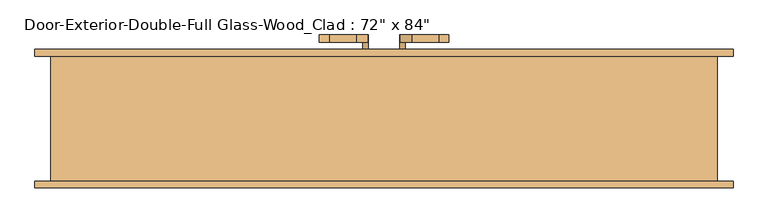
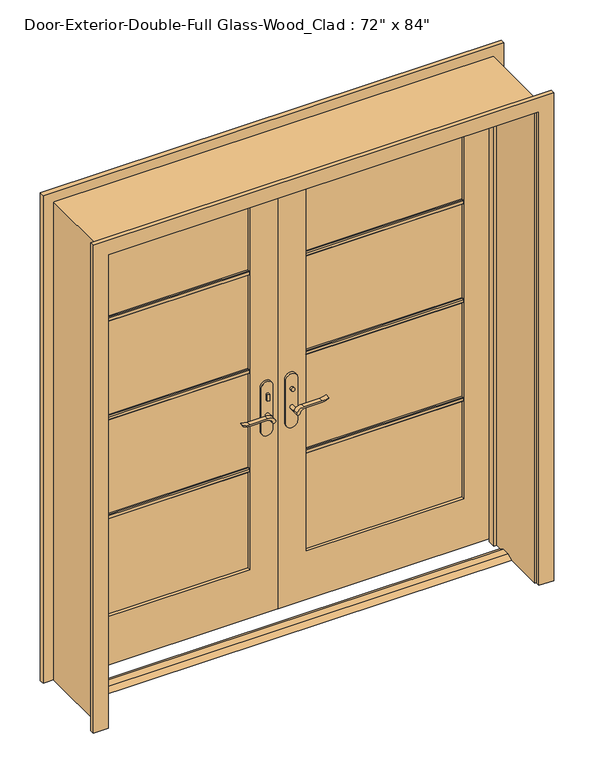
"""IFC4 building model written with IfcOpenShell, lengths in millimetres: door geometry."""

from ifc_helpers import new_model, si_unit, point, frame, frame_2d, origin, place, context, project, spatial, polyline, circle_curve, trimmed, segment, composite_curve, outline, extrude, faceted_brep, source, transform, mapped, element, save


def door_57570b86(model_context):
    return source(origin(), model_context, "Body", "SolidModel", [
        extrude(outline(polyline([(19.05, 12.7), (53.975, 12.7), (79.375, 0.0), (-6.35, 0.0), (19.05, 12.7)])), frame((-914.4, 0.0, 0.0), z_axis=(1.0, 0.0, 0.0), x_axis=(0.0, 1.0, 0.0)), (0.0, 0.0, 1.0), 1828.8),
        extrude(outline(polyline([(-47.4019111, 118.1125), (-57.4019111, 118.1125), (-57.4019111, 128.1125), (-47.4019111, 128.1125), (-47.4019111, 118.1125)])), frame((0.0, 0.0, 981.9), z_axis=(0.0, 0.0, 1.0), x_axis=(1.0, 0.0, 0.0)), (0.0, 0.0, 1.0), 30.0),
        extrude(outline(composite_curve([segment(trimmed(circle_curve(frame_2d((996.9, -52.4019111)), 8.0), [point((996.9, -60.4019111))], [point((996.9, -44.4019111))], False, "CARTESIAN"), True, "CONTINUOUS"), segment(trimmed(circle_curve(frame_2d((996.9, -52.4019111)), 8.0), [point((996.9, -44.4019111))], [point((996.9, -60.4019111))], False, "CARTESIAN"), True, "CONTINUOUS")], self_intersect=False)), frame((0.0, 183.0375, 0.0), z_axis=(0.0, 1.0, 0.0), x_axis=(0.0, 0.0, 1.0)), (0.0, 0.0, 1.0), 10.0),
        extrude(outline(composite_curve([segment(trimmed(circle_curve(frame_2d((897.1555521, -76.0694241)), 37.2832219), [point((919.0523287, -45.8937749))], [point((934.4, -77.7693445))], False, "CARTESIAN"), True, "CONTINUOUS"), segment(polyline([(934.4, -77.7693445), (934.4, -154.045502)]), True, "CONTINUOUS"), segment(trimmed(circle_curve(frame_2d((1017.6850638, -153.9791202)), 83.2850902), [point((934.4, -154.045502))], [point((939.4, -182.4019111))], True, "CARTESIAN"), True, "CONTINUOUS"), segment(polyline([(939.4, -182.4019111), (936.6135558, -182.4019111)]), True, "CONTINUOUS"), segment(trimmed(circle_curve(frame_2d((986.6709207, -150.4622499)), 59.3791355), [point((936.6135558, -182.4019111))], [point((927.4, -154.045502))], False, "CARTESIAN"), True, "CONTINUOUS"), segment(polyline([(927.4, -154.045502), (927.4, -77.7881013)]), True, "CONTINUOUS"), segment(trimmed(circle_curve(frame_2d((909.2738613, -77.7881013)), 18.1261387), [point((927.4, -77.7881013))], [point((914.4, -60.4019111))], True, "CARTESIAN"), True, "CONTINUOUS"), segment(trimmed(circle_curve(frame_2d((914.4, -52.4019111)), 8.0), [point((914.4, -60.4019111))], [point((919.0523287, -45.8937749))], False, "CARTESIAN"), True, "CONTINUOUS")], self_intersect=False)), frame((0.0, 78.1125, 0.0), z_axis=(0.0, 1.0, 0.0), x_axis=(0.0, 0.0, 1.0)), (0.0, 0.0, 1.0), 20.0),
        extrude(outline(composite_curve([segment(trimmed(circle_curve(frame_2d((914.4, -52.4019111)), 8.0), [point((914.3999903, -60.4019111))], [point((919.0523287, -45.8937749))], False, "CARTESIAN"), True, "CONTINUOUS"), segment(trimmed(circle_curve(frame_2d((897.1555521, -76.0694241)), 37.2832219), [point((919.0523287, -45.8937749))], [point((934.4, -77.7693445))], False, "CARTESIAN"), True, "CONTINUOUS"), segment(polyline([(934.4, -77.7693445), (934.4, -154.045502)]), True, "CONTINUOUS"), segment(trimmed(circle_curve(frame_2d((1017.6850638, -153.9791202)), 83.2850902), [point((934.4, -154.045502))], [point((939.4, -182.4019111))], True, "CARTESIAN"), True, "CONTINUOUS"), segment(polyline([(939.4, -182.4019111), (936.6135558, -182.4019111)]), True, "CONTINUOUS"), segment(trimmed(circle_curve(frame_2d((986.6709207, -150.4622499)), 59.3791355), [point((936.6135558, -182.4019111))], [point((927.4, -154.045502))], False, "CARTESIAN"), True, "CONTINUOUS"), segment(polyline([(927.4, -154.045502), (927.4, -77.788099)]), True, "CONTINUOUS"), segment(trimmed(circle_curve(frame_2d((909.2738682, -77.788099)), 18.1261318), [point((927.4, -77.788099))], [point((914.3999903, -60.4019111))], True, "CARTESIAN"), True, "CONTINUOUS")], self_intersect=False)), frame((0.0, 213.0375, 0.0), z_axis=(0.0, 1.0, 0.0), x_axis=(0.0, 0.0, 1.0)), (0.0, 0.0, 1.0), 20.0),
        extrude(outline(composite_curve([segment(trimmed(circle_curve(frame_2d((914.4, -52.4019111)), 8.0), [point((914.4, -60.4019111))], [point((914.4, -44.4019111))], False, "CARTESIAN"), True, "CONTINUOUS"), segment(trimmed(circle_curve(frame_2d((914.4, -52.4019111)), 8.0), [point((914.4, -44.4019111))], [point((914.4, -60.4019111))], False, "CARTESIAN"), True, "CONTINUOUS")], self_intersect=False)), frame((0.0, 98.1125, 0.0), z_axis=(0.0, 1.0, 0.0), x_axis=(0.0, 0.0, 1.0)), (0.0, 0.0, 1.0), 30.0),
        extrude(outline(composite_curve([segment(trimmed(circle_curve(frame_2d((914.4, -52.4019111)), 8.0), [point((914.4, -60.4019111))], [point((914.4, -44.4019111))], False, "CARTESIAN"), True, "CONTINUOUS"), segment(trimmed(circle_curve(frame_2d((914.4, -52.4019111)), 8.0), [point((914.4, -44.4019111))], [point((914.4, -60.4019111))], False, "CARTESIAN"), True, "CONTINUOUS")], self_intersect=False)), frame((0.0, 183.0375, 0.0), z_axis=(0.0, 1.0, 0.0), x_axis=(0.0, 0.0, 1.0)), (0.0, 0.0, 1.0), 30.0),
        extrude(outline(composite_curve([segment(polyline([(844.4, -27.4019111), (1039.4, -27.4019111)]), True, "CONTINUOUS"), segment(trimmed(circle_curve(frame_2d((1039.4, -52.4019111)), 25.0), [point((1039.4, -27.4019111))], [point((1039.4, -77.4019111))], False, "CARTESIAN"), True, "CONTINUOUS"), segment(polyline([(1039.4, -77.4019111), (844.4, -77.4019111)]), True, "CONTINUOUS"), segment(trimmed(circle_curve(frame_2d((844.4, -52.4019111)), 25.0), [point((844.4, -77.4019111))], [point((844.4, -27.4019111))], False, "CARTESIAN"), True, "CONTINUOUS")], self_intersect=False)), frame((0.0, 128.1125, 0.0), z_axis=(0.0, 1.0, 0.0), x_axis=(0.0, 0.0, 1.0)), (0.0, 0.0, 1.0), 10.0),
        extrude(outline(composite_curve([segment(polyline([(844.4, -27.4019111), (1039.4, -27.4019111)]), True, "CONTINUOUS"), segment(trimmed(circle_curve(frame_2d((1039.4, -52.4019111)), 25.0), [point((1039.4, -27.4019111))], [point((1039.4, -77.4019111))], False, "CARTESIAN"), True, "CONTINUOUS"), segment(polyline([(1039.4, -77.4019111), (844.4, -77.4019111)]), True, "CONTINUOUS"), segment(trimmed(circle_curve(frame_2d((844.4, -52.4019111)), 25.0), [point((844.4, -77.4019111))], [point((844.4, -27.4019111))], False, "CARTESIAN"), True, "CONTINUOUS")], self_intersect=False)), frame((0.0, 173.0375, 0.0), z_axis=(0.0, 1.0, 0.0), x_axis=(0.0, 0.0, 1.0)), (0.0, 0.0, 1.0), 10.0),
        extrude(outline(polyline([(47.3875, 193.0375), (57.3875, 193.0375), (57.3875, 183.0375), (47.3875, 183.0375), (47.3875, 193.0375)])), frame((0.0, 0.0, 981.9), z_axis=(0.0, 0.0, 1.0), x_axis=(1.0, 0.0, 0.0)), (0.0, 0.0, 1.0), 30.0),
        extrude(outline(composite_curve([segment(trimmed(circle_curve(frame_2d((996.9, 52.3875)), 8.0), [point((996.9, 60.3875))], [point((996.9, 44.3875))], False, "CARTESIAN"), True, "CONTINUOUS"), segment(trimmed(circle_curve(frame_2d((996.9, 52.3875)), 8.0), [point((996.9, 44.3875))], [point((996.9, 60.3875))], False, "CARTESIAN"), True, "CONTINUOUS")], self_intersect=False)), frame((0.0, 118.1125, 0.0), z_axis=(0.0, 1.0, 0.0), x_axis=(0.0, 0.0, 1.0)), (0.0, 0.0, 1.0), 10.0),
        extrude(outline(composite_curve([segment(trimmed(circle_curve(frame_2d((914.4, 52.3875)), 8.0), [point((919.0523287, 45.8793637))], [point((914.4, 60.3875))], False, "CARTESIAN"), True, "CONTINUOUS"), segment(trimmed(circle_curve(frame_2d((909.2738613, 77.7736901)), 18.1261387), [point((914.4, 60.3875))], [point((927.4, 77.7736901))], True, "CARTESIAN"), True, "CONTINUOUS"), segment(polyline([(927.4, 77.7736901), (927.4, 154.0310909)]), True, "CONTINUOUS"), segment(trimmed(circle_curve(frame_2d((986.6709207, 150.4478388)), 59.3791355), [point((927.4, 154.0310909))], [point((936.6135558, 182.3875))], False, "CARTESIAN"), True, "CONTINUOUS"), segment(polyline([(936.6135558, 182.3875), (939.4, 182.3875)]), True, "CONTINUOUS"), segment(trimmed(circle_curve(frame_2d((1017.6850638, 153.9647091)), 83.2850902), [point((939.4, 182.3875))], [point((934.4, 154.0310909))], True, "CARTESIAN"), True, "CONTINUOUS"), segment(polyline([(934.4, 154.0310909), (934.4, 77.7549333)]), True, "CONTINUOUS"), segment(trimmed(circle_curve(frame_2d((897.1555521, 76.0550129)), 37.2832219), [point((934.4, 77.7549333))], [point((919.0523287, 45.8793637))], False, "CARTESIAN"), True, "CONTINUOUS")], self_intersect=False)), frame((0.0, 213.0375, 0.0), z_axis=(0.0, 1.0, 0.0), x_axis=(0.0, 0.0, 1.0)), (0.0, 0.0, 1.0), 20.0),
        extrude(outline(composite_curve([segment(trimmed(circle_curve(frame_2d((909.2738682, 77.7736878)), 18.1261318), [point((914.3999903, 60.3875))], [point((927.4, 77.7736878))], True, "CARTESIAN"), True, "CONTINUOUS"), segment(polyline([(927.4, 77.7736878), (927.4, 154.0310909)]), True, "CONTINUOUS"), segment(trimmed(circle_curve(frame_2d((986.6709207, 150.4478388)), 59.3791355), [point((927.4, 154.0310909))], [point((936.6135558, 182.3875))], False, "CARTESIAN"), True, "CONTINUOUS"), segment(polyline([(936.6135558, 182.3875), (939.4, 182.3875)]), True, "CONTINUOUS"), segment(trimmed(circle_curve(frame_2d((1017.6850638, 153.9647091)), 83.2850902), [point((939.4, 182.3875))], [point((934.4, 154.0310909))], True, "CARTESIAN"), True, "CONTINUOUS"), segment(polyline([(934.4, 154.0310909), (934.4, 77.7549333)]), True, "CONTINUOUS"), segment(trimmed(circle_curve(frame_2d((897.1555521, 76.0550129)), 37.2832219), [point((934.4, 77.7549333))], [point((919.0523287, 45.8793637))], False, "CARTESIAN"), True, "CONTINUOUS"), segment(trimmed(circle_curve(frame_2d((914.4, 52.3875)), 8.0), [point((919.0523287, 45.8793637))], [point((914.3999903, 60.3875))], False, "CARTESIAN"), True, "CONTINUOUS")], self_intersect=False)), frame((0.0, 78.1125, 0.0), z_axis=(0.0, 1.0, 0.0), x_axis=(0.0, 0.0, 1.0)), (0.0, 0.0, 1.0), 20.0),
        extrude(outline(composite_curve([segment(trimmed(circle_curve(frame_2d((914.4, 52.3875)), 8.0), [point((914.4, 60.3875))], [point((914.4, 44.3875))], False, "CARTESIAN"), True, "CONTINUOUS"), segment(trimmed(circle_curve(frame_2d((914.4, 52.3875)), 8.0), [point((914.4, 44.3875))], [point((914.4, 60.3875))], False, "CARTESIAN"), True, "CONTINUOUS")], self_intersect=False)), frame((0.0, 183.0375, 0.0), z_axis=(0.0, 1.0, 0.0), x_axis=(0.0, 0.0, 1.0)), (0.0, 0.0, 1.0), 30.0),
        extrude(outline(composite_curve([segment(trimmed(circle_curve(frame_2d((914.4, 52.3875)), 8.0), [point((914.4, 60.3875))], [point((914.4, 44.3875))], False, "CARTESIAN"), True, "CONTINUOUS"), segment(trimmed(circle_curve(frame_2d((914.4, 52.3875)), 8.0), [point((914.4, 44.3875))], [point((914.4, 60.3875))], False, "CARTESIAN"), True, "CONTINUOUS")], self_intersect=False)), frame((0.0, 98.1125, 0.0), z_axis=(0.0, 1.0, 0.0), x_axis=(0.0, 0.0, 1.0)), (0.0, 0.0, 1.0), 30.0),
        extrude(outline(composite_curve([segment(trimmed(circle_curve(frame_2d((844.4, 52.3875)), 25.0), [point((844.4, 27.3875))], [point((844.4, 77.3875))], False, "CARTESIAN"), True, "CONTINUOUS"), segment(polyline([(844.4, 77.3875), (1039.4, 77.3875)]), True, "CONTINUOUS"), segment(trimmed(circle_curve(frame_2d((1039.4, 52.3875)), 25.0), [point((1039.4, 77.3875))], [point((1039.4, 27.3875))], False, "CARTESIAN"), True, "CONTINUOUS"), segment(polyline([(1039.4, 27.3875), (844.4, 27.3875)]), True, "CONTINUOUS")], self_intersect=False)), frame((0.0, 173.0375, 0.0), z_axis=(0.0, 1.0, 0.0), x_axis=(0.0, 0.0, 1.0)), (0.0, 0.0, 1.0), 10.0),
        extrude(outline(composite_curve([segment(trimmed(circle_curve(frame_2d((844.4, 52.3875)), 25.0), [point((844.4, 27.3875))], [point((844.4, 77.3875))], False, "CARTESIAN"), True, "CONTINUOUS"), segment(polyline([(844.4, 77.3875), (1039.4, 77.3875)]), True, "CONTINUOUS"), segment(trimmed(circle_curve(frame_2d((1039.4, 52.3875)), 25.0), [point((1039.4, 77.3875))], [point((1039.4, 27.3875))], False, "CARTESIAN"), True, "CONTINUOUS"), segment(polyline([(1039.4, 27.3875), (844.4, 27.3875)]), True, "CONTINUOUS")], self_intersect=False)), frame((0.0, 128.1125, 0.0), z_axis=(0.0, 1.0, 0.0), x_axis=(0.0, 0.0, 1.0)), (0.0, 0.0, 1.0), 10.0),
        extrude(outline(polyline([(152.0825, 1578.371875), (152.0825, 1559.321875), (145.7325, 1559.321875), (142.5575, 1562.496875), (142.5575, 1575.196875), (145.7325, 1578.371875), (152.0825, 1578.371875)])), frame((120.65, 0.0, 0.0), z_axis=(1.0, 0.0, 0.0), x_axis=(0.0, 1.0, 0.0)), (0.0, 0.0, 1.0), 673.1),
        extrude(outline(polyline([(152.0825, 1132.68125), (152.0825, 1113.63125), (145.7325, 1113.63125), (142.5575, 1116.80625), (142.5575, 1129.50625), (145.7325, 1132.68125), (152.0825, 1132.68125)])), frame((120.65, 0.0, 0.0), z_axis=(1.0, 0.0, 0.0), x_axis=(0.0, 1.0, 0.0)), (0.0, 0.0, 1.0), 673.1),
        extrude(outline(polyline([(152.0825, 686.990625), (152.0825, 667.940625), (145.7325, 667.940625), (142.5575, 671.115625), (142.5575, 683.815625), (145.7325, 686.990625), (152.0825, 686.990625)])), frame((120.65, 0.0, 0.0), z_axis=(1.0, 0.0, 0.0), x_axis=(0.0, 1.0, 0.0)), (0.0, 0.0, 1.0), 673.1),
        extrude(outline(polyline([(159.0675, 1578.371875), (165.4175, 1578.371875), (168.5925, 1575.196875), (168.5925, 1562.496875), (165.4175, 1559.321875), (159.0675, 1559.321875), (159.0675, 1578.371875)])), frame((-793.75, 0.0, 0.0), z_axis=(1.0, 0.0, 0.0), x_axis=(0.0, 1.0, 0.0)), (0.0, 0.0, 1.0), 673.1),
        extrude(outline(polyline([(159.0675, 1132.68125), (165.4175, 1132.68125), (168.5925, 1129.50625), (168.5925, 1116.80625), (165.4175, 1113.63125), (159.0675, 1113.63125), (159.0675, 1132.68125)])), frame((-793.75, 0.0, 0.0), z_axis=(1.0, 0.0, 0.0), x_axis=(0.0, 1.0, 0.0)), (0.0, 0.0, 1.0), 673.1),
        extrude(outline(polyline([(159.0675, 686.990625), (165.4175, 686.990625), (168.5925, 683.815625), (168.5925, 671.115625), (165.4175, 667.940625), (159.0675, 667.940625), (159.0675, 686.990625)])), frame((-793.75, 0.0, 0.0), z_axis=(1.0, 0.0, 0.0), x_axis=(0.0, 1.0, 0.0)), (0.0, 0.0, 1.0), 673.1),
        extrude(outline(polyline([(159.0675, 1578.371875), (165.4175, 1578.371875), (168.5925, 1575.196875), (168.5925, 1562.496875), (165.4175, 1559.321875), (159.0675, 1559.321875), (159.0675, 1578.371875)])), frame((120.65, 0.0, 0.0), z_axis=(1.0, 0.0, 0.0), x_axis=(0.0, 1.0, 0.0)), (0.0, 0.0, 1.0), 673.1),
        extrude(outline(polyline([(159.0675, 1132.68125), (165.4175, 1132.68125), (168.5925, 1129.50625), (168.5925, 1116.80625), (165.4175, 1113.63125), (159.0675, 1113.63125), (159.0675, 1132.68125)])), frame((120.65, 0.0, 0.0), z_axis=(1.0, 0.0, 0.0), x_axis=(0.0, 1.0, 0.0)), (0.0, 0.0, 1.0), 673.1),
        extrude(outline(polyline([(159.0675, 686.990625), (165.4175, 686.990625), (168.5925, 683.815625), (168.5925, 671.115625), (165.4175, 667.940625), (159.0675, 667.940625), (159.0675, 686.990625)])), frame((120.65, 0.0, 0.0), z_axis=(1.0, 0.0, 0.0), x_axis=(0.0, 1.0, 0.0)), (0.0, 0.0, 1.0), 673.1),
        extrude(outline(polyline([(152.0825, 1578.371875), (152.0825, 1559.321875), (145.7325, 1559.321875), (142.5575, 1562.496875), (142.5575, 1575.196875), (145.7325, 1578.371875), (152.0825, 1578.371875)])), frame((-793.75, 0.0, 0.0), z_axis=(1.0, 0.0, 0.0), x_axis=(0.0, 1.0, 0.0)), (0.0, 0.0, 1.0), 673.1),
        extrude(outline(polyline([(152.0825, 1132.68125), (152.0825, 1113.63125), (145.7325, 1113.63125), (142.5575, 1116.80625), (142.5575, 1129.50625), (145.7325, 1132.68125), (152.0825, 1132.68125)])), frame((-793.75, 0.0, 0.0), z_axis=(1.0, 0.0, 0.0), x_axis=(0.0, 1.0, 0.0)), (0.0, 0.0, 1.0), 673.1),
        extrude(outline(polyline([(152.0825, 686.990625), (152.0825, 667.940625), (145.7325, 667.940625), (142.5575, 671.115625), (142.5575, 683.815625), (145.7325, 686.990625), (152.0825, 686.990625)])), frame((-793.75, 0.0, 0.0), z_axis=(1.0, 0.0, 0.0), x_axis=(0.0, 1.0, 0.0)), (0.0, 0.0, 1.0), 673.1),
        extrude(outline(polyline([(0.0, 920.75), (0.0, 984.25), (2203.45, 984.25), (2203.45, -984.25), (0.0, -984.25), (0.0, -920.75), (2139.95, -920.75), (2139.95, 920.75), (0.0, 920.75)])), frame((0.0, 173.0375, 0.0), z_axis=(0.0, 1.0, 0.0), x_axis=(0.0, 0.0, 1.0)), (0.0, 0.0, 1.0), 19.05),
        extrude(outline(polyline([(0.0, 920.75), (0.0, 984.25), (2203.45, 984.25), (2203.45, -984.25), (0.0, -984.25), (0.0, -920.75), (2139.95, -920.75), (2139.95, 920.75), (0.0, 920.75)])), frame((0.0, -198.4375, 0.0), z_axis=(0.0, 1.0, 0.0), x_axis=(0.0, 0.0, 1.0)), (0.0, 0.0, 1.0), 19.05),
        extrude(outline(polyline([(12.7, 914.4), (2133.6, 914.4), (2133.6, 1.5875), (12.7, 1.5875), (12.7, 914.4)]), holes=[polyline([(2014.5375, 120.65), (2014.5375, 793.75), (231.775, 793.75), (231.775, 120.65), (2014.5375, 120.65)])]), frame((0.0, 138.1125, 0.0), z_axis=(0.0, 1.0, 0.0), x_axis=(0.0, 0.0, 1.0)), (0.0, 0.0, 1.0), 34.925),
        extrude(outline(polyline([(2133.6, -914.4), (12.7, -914.4), (12.7, -1.6019111), (2133.6, -1.6019111), (2133.6, -914.4)]), holes=[polyline([(231.775, -793.75), (2014.5375, -793.75), (2014.5375, -120.65), (231.775, -120.65), (231.775, -793.75)])]), frame((0.0, 138.1125, 0.0), z_axis=(0.0, 1.0, 0.0), x_axis=(0.0, 0.0, 1.0)), (0.0, 0.0, 1.0), 34.925),
        faceted_brep([(939.8, 173.0375, 0.0), (939.8, -179.3875, 0.0), (914.4, -179.3875, 0.0), (914.4, 103.1875, 0.0), (901.7, 103.1875, 0.0), (901.7, 138.1125, 0.0), (914.4, 138.1125, 0.0), (914.4, 173.0375, 0.0), (939.8, 173.0375, 2159.0), (939.8, -179.3875, 2159.0), (-939.8, -179.3875, 2159.0), (-939.8, -179.3875, 0.0), (-914.4, -179.3875, 0.0), (-914.4, -179.3875, 2133.6), (914.4, -179.3875, 2133.6), (914.4, 103.1875, 2133.6), (-914.4, 103.1875, 2133.6), (-914.4, 103.1875, 0.0), (-901.7, 103.1875, 0.0), (-901.7, 103.1875, 2120.9), (901.7, 103.1875, 2120.9), (901.7, 138.1125, 2120.9), (1.5875, 138.1125, 2120.9), (-1.6019111, 138.1125, 2120.9), (-901.7, 138.1125, 2120.9), (-901.7, 138.1125, 0.0), (-914.4, 138.1125, 0.0), (-914.4, 138.1125, 2133.6), (-1.6019111, 138.1125, 2133.6), (1.5875, 138.1125, 2133.6), (914.4, 138.1125, 2133.6), (914.4, 173.0375, 2133.6), (1.5875, 173.0375, 2133.6), (-1.6019111, 173.0375, 2133.6), (-914.4, 173.0375, 2133.6), (-914.4, 173.0375, 0.0), (-939.8, 173.0375, 0.0), (-939.8, 173.0375, 2159.0)], [[[0, 1, 2, 3, 4, 5, 6, 7]], [[1, 0, 8, 9]], [[2, 1, 9, 10, 11, 12, 13, 14]], [[3, 2, 14, 15]], [[4, 3, 15, 16, 17, 18, 19, 20]], [[5, 4, 20, 21]], [[6, 5, 21, 22, 23, 24, 25, 26, 27, 28, 29, 30]], [[7, 6, 30, 31]], [[0, 7, 31, 32, 33, 34, 35, 36, 37, 8]], [[9, 8, 37, 10]], [[14, 13, 16, 15]], [[20, 19, 24, 23, 22, 21]], [[31, 30, 29, 28, 27, 34, 33, 32]], [[12, 11, 36, 35, 26, 25, 18, 17]], [[11, 10, 37, 36]], [[13, 12, 17, 16]], [[19, 18, 25, 24]], [[27, 26, 35, 34]]]),
        extrude(outline(polyline([(793.75, 152.0825), (120.65, 152.0825), (120.65, 159.0675), (793.75, 159.0675), (793.75, 152.0825)])), frame((0.0, 0.0, 231.775), z_axis=(0.0, 0.0, 1.0), x_axis=(1.0, 0.0, 0.0)), (0.0, 0.0, 1.0), 1782.7625),
        extrude(outline(polyline([(-120.65, 152.0825), (-793.75, 152.0825), (-793.75, 159.0675), (-120.65, 159.0675), (-120.65, 152.0825)])), frame((0.0, 0.0, 231.775), z_axis=(0.0, 0.0, 1.0), x_axis=(1.0, 0.0, 0.0)), (0.0, 0.0, 1.0), 1782.7625),
    ])


if __name__ == "__main__":
    model = new_model("IFC4")
    model_context = context("Model", 3, world=origin())
    ifc_project = project(units=[si_unit("LENGTHUNIT", "METRE", prefix="MILLI")], contexts=[model_context])
    site = spatial("IfcSite", under=ifc_project)
    building = spatial("IfcBuilding", under=site)
    placement = place(None, origin())
    door_shape = door_57570b86(model_context)
    element("IfcDoor", 1, ObjectType="Door-Exterior-Double-Full Glass-Wood_Clad : 72\" x 84\"", at=placement, inside=building, context=model_context, shape_type="MappedRepresentation", body=[
        mapped(door_shape, transform((0.0, 0.0, 0.0), x_axis=(1.0, 0.0, 0.0), y_axis=(0.0, 1.0, 0.0), z_axis=(0.0, 0.0, 1.0))),
    ])
    save(model, "model.ifc")

# Revit data of these elements
# Type "Door-Exterior-Double-Full Glass-Wood_Clad : 72\" x 84\""
#   Type Mark = "24"
#   Assembly Code = "B2030100"
#   Analytic Construction = "French door, wood frame with double glass"
#   Top Rail = 0' - 4 11/16"
#   Threshold Offset [instance default] = 0' - 0 1/2"
#   Thickness = 0' - 1 3/8"
#   Thermal Resistance (R) = 1.9158 (h·ft²·°F)/BTU
#   Swing Angle [instance default] = 90.0000°
#   Stiles = 0' - 4 3/4"
#   Rough Width = 6' - 2"
#   Rough Height = 7' - 1"
#   Panel Width = 3' - 0"
#   Door Offset [instance default] = 0' - 0"
#   Height = 7' - 0"
#   Width = 6' - 0"
#   Heat Transfer Coefficient (U) = 0.5220 BTU/(h·ft²·°F)
#   Bottom Rail = 0' - 9 1/8"
#   Exterior Trim [instance default] = yes
#   Threshold [instance default] = yes
#   Show Grill [instance default] = yes
#   Function = 1
#   Trim Material = Cherry
#   Threshold Material = Cherry
#   Panel Material = Cherry
#   Glazing = Glass
#   Frame Material = Cherry
#   Door Handle Material = Aluminum
#   Visual Light Transmittance = 0
#   Solar Heat Gain Coefficient = 0
#   Wall Closure = (empty or 0)
#   Construction Type = (empty or 0)
# Element 1 (IfcDoor, "Door-Exterior-Double-Full Glass-Wood_Clad : 72\" x 84\"")
#   Materials on its faces: "Cherry", "Aluminum", "Glass"
# Materials
#   "Cherry": class "Wood", colour RGB 226 177 128, transparency 0, Description = "Prunus Serotina", Cost = 0
#   "Glass": class "Glass", colour RGB 0 128 192, transparency 0.75, Description = "Soda Lime Glass", Cost = 0
#   "Aluminum": class "Metal", colour RGB 247 247 247, transparency 0, Description = "Aluminum 6061", Cost = 0
